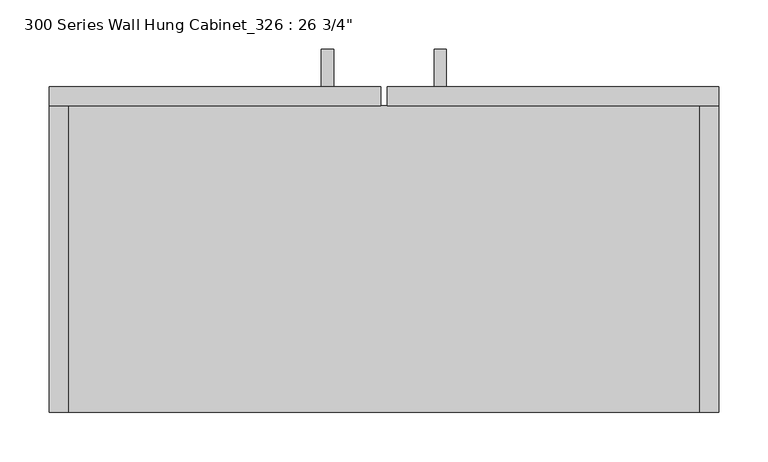
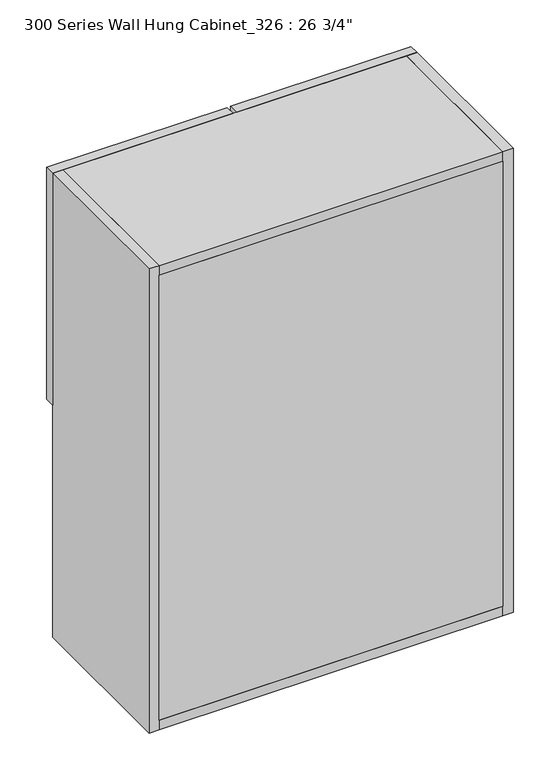
"""IFC4 building model written with IfcOpenShell, lengths in millimetres: furniture geometry."""

from ifc_helpers import new_model, si_unit, frame, origin, place, context, project, spatial, polyline, outline, extrude, source, transform, mapped, element, save


def furniture_52e44281(model_context):
    return source(origin(), model_context, "Body", "SweptSolid", [
        extrude(outline(polyline([(390.525, 1809.7425373), (390.525, 1822.4121874), (428.6060937, 1822.4121874), (428.6060937, 1727.2), (390.525, 1727.2), (390.525, 1739.8696501), (415.9364436, 1739.8696501), (415.9364436, 1809.7425373), (390.525, 1809.7425373)])), frame((50.8, 0.0, 0.0), z_axis=(1.0, 0.0, 0.0), x_axis=(0.0, 1.0, 0.0)), (0.0, 0.0, 1.0), 12.4065288),
        extrude(outline(polyline([(390.525, 1809.7425373), (390.525, 1822.4121874), (428.6060937, 1822.4121874), (428.6060937, 1727.2), (390.525, 1727.2), (390.525, 1739.8696501), (415.9364436, 1739.8696501), (415.9364436, 1809.7425373), (390.525, 1809.7425373)])), frame((-63.5, 0.0, 0.0), z_axis=(1.0, 0.0, 0.0), x_axis=(0.0, 1.0, 0.0)), (0.0, 0.0, 1.0), 12.4065288),
        extrude(outline(polyline([(320.675, 371.475), (320.675, 79.375), (-320.675, 79.375), (-320.675, 371.475), (320.675, 371.475)])), frame((0.0, 0.0, 1676.4), z_axis=(0.0, 0.0, 1.0), x_axis=(1.0, 0.0, 0.0)), (0.0, 0.0, 1.0), 19.05),
        extrude(outline(polyline([(320.675, 60.325), (-320.675, 60.325), (-320.675, 79.375), (320.675, 79.375), (320.675, 60.325)])), frame((0.0, 0.0, 1238.25), z_axis=(0.0, 0.0, 1.0), x_axis=(1.0, 0.0, 0.0)), (0.0, 0.0, 1.0), 876.3),
        extrude(outline(polyline([(-3.175, 371.475), (-339.725, 371.475), (-339.725, 390.525), (-3.175, 390.525), (-3.175, 371.475)])), frame((0.0, 0.0, 1676.4), z_axis=(0.0, 0.0, 1.0), x_axis=(1.0, 0.0, 0.0)), (0.0, 0.0, 1.0), 457.2),
        extrude(outline(polyline([(339.725, 371.475), (3.175, 371.475), (3.175, 390.525), (339.725, 390.525), (339.725, 371.475)])), frame((0.0, 0.0, 1676.4), z_axis=(0.0, 0.0, 1.0), x_axis=(1.0, 0.0, 0.0)), (0.0, 0.0, 1.0), 457.2),
        extrude(outline(polyline([(-339.725, 60.325), (-339.725, 371.475), (-320.675, 371.475), (-320.675, 60.325), (-339.725, 60.325)])), frame((0.0, 0.0, 1219.2), z_axis=(0.0, 0.0, 1.0), x_axis=(1.0, 0.0, 0.0)), (0.0, 0.0, 1.0), 914.4),
        extrude(outline(polyline([(320.675, 60.325), (320.675, 371.475), (339.725, 371.475), (339.725, 60.325), (320.675, 60.325)])), frame((0.0, 0.0, 1219.2), z_axis=(0.0, 0.0, 1.0), x_axis=(1.0, 0.0, 0.0)), (0.0, 0.0, 1.0), 914.4),
        extrude(outline(polyline([(320.675, 371.475), (320.675, 60.325), (-320.675, 60.325), (-320.675, 371.475), (320.675, 371.475)])), frame((0.0, 0.0, 2114.55), z_axis=(0.0, 0.0, 1.0), x_axis=(1.0, 0.0, 0.0)), (0.0, 0.0, 1.0), 19.05),
        extrude(outline(polyline([(320.675, 371.475), (320.675, 60.325), (-320.675, 60.325), (-320.675, 371.475), (320.675, 371.475)])), frame((0.0, 0.0, 1219.2), z_axis=(0.0, 0.0, 1.0), x_axis=(1.0, 0.0, 0.0)), (0.0, 0.0, 1.0), 19.05),
    ])


if __name__ == "__main__":
    model = new_model("IFC4")
    model_context = context("Model", 3, world=origin())
    ifc_project = project(units=[si_unit("LENGTHUNIT", "METRE", prefix="MILLI")], contexts=[model_context])
    site = spatial("IfcSite", under=ifc_project)
    building = spatial("IfcBuilding", under=site)
    placement = place(None, origin())
    furniture_shape = furniture_52e44281(model_context)
    element("IfcFurniture", 1, ObjectType="300 Series Wall Hung Cabinet_326 : 26 3/4\"", at=placement, inside=building, context=model_context, shape_type="MappedRepresentation", body=[
        mapped(furniture_shape, transform((0.0, 0.0, 0.0), x_axis=(1.0, 0.0, 0.0), y_axis=(0.0, 1.0, 0.0), z_axis=(0.0, 0.0, 1.0))),
    ])
    save(model, "model.ifc")

# Revit data of these elements
# Type "300 Series Wall Hung Cabinet_326 : 26 3/4\""
#   URL = "www.wicnet.org/manual_sections.asp"
#   Model = "326"
#   Manufacturer = "Woodwork Institute"
#   Content Creator URL = "www.AECcontent.com"
#   Content Creator = "AECcontent"
#   Description = "Wall Hung Cabinet"
#   Assembly Code = "E2010200"
#   Width = 2' - 2 3/4"
#   Top of Cabinet = 7' - 0"
#   Height = 3' - 0"
#   Depth = 1' - 1"
#   Top Panel Material = none
#   Side Panel Material = none
#   Shelf Panel Material = none
#   Back Panel Material = none
#   Door Panel Material = none
# Element 1 (IfcFurniture, "300 Series Wall Hung Cabinet_326 : 26 3/4\"")
#   Materials on its faces: "CASEWORK"
# Materials
#   "CASEWORK": class "Generic", colour RGB 181 181 181, transparency 0, Cost = 0
